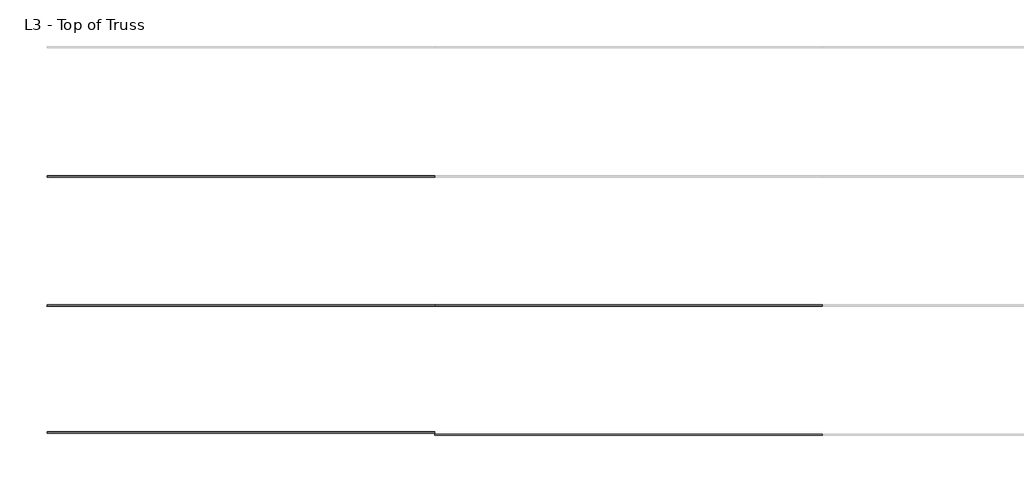
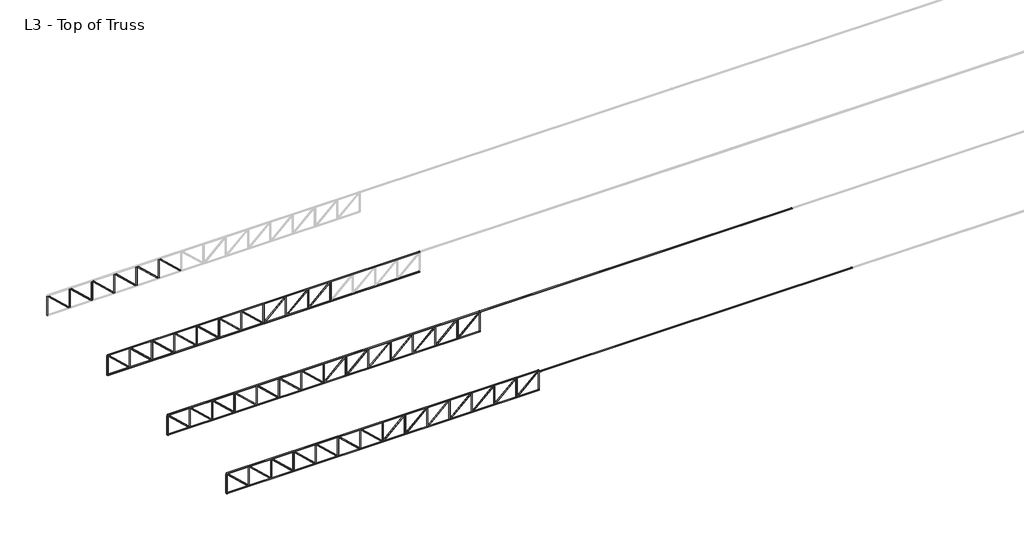
# One storey, part 1 of 2: 99 beams.
"""IFC4 building model written with IfcOpenShell, lengths in millimetres."""

import ifcopenshell
import ifcopenshell.guid

model = None  # the IFC model being written
_history = None  # IfcOwnerHistory: only IFC2X3 demands one
_inside = {}  # id of a spatial element -> (the spatial element, [elements in it])
_under = {}  # id of a project, library or spatial element -> (it, [spatial elements below it])
_declared = {}  # id of a project -> (the project, [libraries it declares])
_typed = {}  # id of a type object -> (the type object, [elements of that type])
_made_of = {}  # id of a material, layer set ... -> (it, [elements and type objects made of it])


def new_model(schema):
    """Start an empty IFC model of exactly this schema.

    Asked for "IFC4X3", IfcOpenShell would pick the latest addendum, in which some entities
    have other attributes; the version numbers below select the first issue.
    IFC2X3 requires an IfcOwnerHistory on every rooted entity: one is made here for all.
    """
    global model, _history
    if schema == "IFC4X3":
        model = ifcopenshell.file(schema_version=(4, 3, 0, 0))
    else:
        model = ifcopenshell.file(schema=schema)
    _inside.clear()
    _under.clear()
    _declared.clear()
    _typed.clear()
    _made_of.clear()
    _history = None
    if model.schema == "IFC2X3":
        org = make("IfcOrganization", Name="unknown")
        user = make(
            "IfcPersonAndOrganization",
            ThePerson=make("IfcPerson", FamilyName="unknown"),
            TheOrganization=org,
        )
        app = make(
            "IfcApplication",
            ApplicationDeveloper=org,
            Version="unknown",
            ApplicationFullName="unknown",
            ApplicationIdentifier="unknown",
        )
        _history = make(
            "IfcOwnerHistory",
            OwningUser=user,
            OwningApplication=app,
            ChangeAction="ADDED",
            CreationDate=0,
        )
    return model


def make(cls, **values):
    """One entity of the class cls with the attributes given. An attribute that is None is left unset."""
    return model.create_entity(
        cls, **{name: value for name, value in values.items() if value is not None}
    )


def rooted(cls, **values):
    """An entity with a GlobalId (a new one), such as an element, a storey or a relation."""
    return make(cls, GlobalId=ifcopenshell.guid.new(), OwnerHistory=_history, **values)


def si_unit(unit_type, name, prefix=None):
    """IfcSIUnit, for example si_unit("LENGTHUNIT", "METRE", prefix="MILLI")."""
    return make("IfcSIUnit", UnitType=unit_type, Prefix=prefix, Name=name)


def assignment(units):
    """IfcUnitAssignment: the units of a project."""
    return None if units is None else make("IfcUnitAssignment", Units=units)


def point(xyz):
    """IfcCartesianPoint."""
    return None if xyz is None else make("IfcCartesianPoint", Coordinates=xyz)


def direction(xyz):
    """IfcDirection."""
    return None if xyz is None else make("IfcDirection", DirectionRatios=xyz)


def frame(location, z_axis=None, x_axis=None):
    """IfcAxis2Placement3D, a coordinate frame: its origin and axes. An axis left out is left unset."""
    return make(
        "IfcAxis2Placement3D",
        Location=point(location),
        Axis=direction(z_axis),
        RefDirection=direction(x_axis),
    )


def frame_2d(location, x_axis=None):
    """IfcAxis2Placement2D, a coordinate frame in the plane: its origin and x axis."""
    return make(
        "IfcAxis2Placement2D", Location=point(location), RefDirection=direction(x_axis)
    )


def origin():
    """The frame at (0, 0, 0) with its axes left unset."""
    return frame((0.0, 0.0, 0.0))


def origin_2d():
    """The frame at (0, 0) in the plane with its x axis left unset."""
    return frame_2d((0.0, 0.0))


def place(relative_to, where):
    """IfcLocalPlacement: puts the frame where relative to a parent placement (None: the world)."""
    return make(
        "IfcLocalPlacement", PlacementRelTo=relative_to, RelativePlacement=where
    )


def context(
    kind, dimensions, precision=None, world=None, true_north=None, identifier=None
):
    """IfcGeometricRepresentationContext, for example the 3D "Model" context."""
    return make(
        "IfcGeometricRepresentationContext",
        ContextIdentifier=identifier,
        ContextType=kind,
        CoordinateSpaceDimension=dimensions,
        Precision=precision,
        WorldCoordinateSystem=world,
        TrueNorth=true_north,
    )


def project(units=None, contexts=None):
    """IfcProject with its units and contexts."""
    return rooted(
        "IfcProject",
        Name="project",
        RepresentationContexts=contexts,
        UnitsInContext=assignment(units),
    )


def spatial(cls, under=None, at=None, **own):
    """A site, building, storey or space (cls), placed at a placement, below another one or the project."""
    s = rooted(cls, ObjectPlacement=at, **own)
    if under is not None:
        _under.setdefault(under.id(), (under, []))[1].append(s)
    return s


def circle_curve(where, radius):
    """IfcCircle in the frame where."""
    return make("IfcCircle", Position=where, Radius=radius)


def trimmed(basis, trim1, trim2, sense, master):
    """IfcTrimmedCurve: the piece of a basis curve between two trims."""
    return make(
        "IfcTrimmedCurve",
        BasisCurve=basis,
        Trim1=trim1,
        Trim2=trim2,
        SenseAgreement=sense,
        MasterRepresentation=master,
    )


def segment(curve, same_sense, transition):
    """IfcCompositeCurveSegment."""
    return make(
        "IfcCompositeCurveSegment",
        Transition=transition,
        SameSense=same_sense,
        ParentCurve=curve,
    )


def composite_curve(segments, self_intersect=None):
    """IfcCompositeCurve: segments joined end to end."""
    return make("IfcCompositeCurve", Segments=segments, SelfIntersect=self_intersect)


def outline(outer, holes=None, kind="AREA"):
    """IfcArbitraryClosedProfileDef: a profile drawn as a closed curve; with holes, ...WithVoids."""
    if holes is None:
        return make("IfcArbitraryClosedProfileDef", ProfileType=kind, OuterCurve=outer)
    return make(
        "IfcArbitraryProfileDefWithVoids",
        ProfileType=kind,
        OuterCurve=outer,
        InnerCurves=holes,
    )


def extrude(swept, where, along, depth):
    """IfcExtrudedAreaSolid: the profile swept, set in the frame where, extruded along a direction by depth."""
    return make(
        "IfcExtrudedAreaSolid",
        SweptArea=swept,
        Position=where,
        ExtrudedDirection=direction(along),
        Depth=depth,
    )


def shape(context_of_items, identifier, shape_type, items):
    """IfcShapeRepresentation: the items that make up one representation, for example the "Body"."""
    return make(
        "IfcShapeRepresentation",
        ContextOfItems=context_of_items,
        RepresentationIdentifier=identifier,
        RepresentationType=shape_type,
        Items=items,
    )


def source(mapping_origin, context_of_items, identifier, shape_type, items):
    """IfcRepresentationMap: a shape defined once, which mapped items show again and again."""
    return make(
        "IfcRepresentationMap",
        MappingOrigin=mapping_origin,
        MappedRepresentation=shape(context_of_items, identifier, shape_type, items),
    )


def transform(
    local_origin,
    x_axis=None,
    y_axis=None,
    z_axis=None,
    scale=None,
    scale2=None,
    scale3=None,
    uniform=True,
):
    """IfcCartesianTransformationOperator3D, or its non-uniform kind. x_axis, y_axis, z_axis: its Axis1, 2, 3."""
    if uniform:
        return make(
            "IfcCartesianTransformationOperator3D",
            Axis1=direction(x_axis),
            Axis2=direction(y_axis),
            LocalOrigin=point(local_origin),
            Scale=scale,
            Axis3=direction(z_axis),
        )
    return make(
        "IfcCartesianTransformationOperator3DnonUniform",
        Axis1=direction(x_axis),
        Axis2=direction(y_axis),
        LocalOrigin=point(local_origin),
        Scale=scale,
        Axis3=direction(z_axis),
        Scale2=scale2,
        Scale3=scale3,
    )


def mapped(mapping_source, mapping_target):
    """IfcMappedItem: shows the shape of a source again, moved by a transform."""
    return make(
        "IfcMappedItem", MappingSource=mapping_source, MappingTarget=mapping_target
    )


def made_of(thing, what):
    """Note that an element or type object is made of a material, layer set ...; save() writes the relation."""
    if what is not None:
        _made_of.setdefault(what.id(), (what, []))[1].append(thing)
    return thing


def element(
    cls,
    number,
    at=None,
    inside=None,
    cuts=None,
    type_object=None,
    material=None,
    context=None,
    identifier="Body",
    shape_type=None,
    held_by="IfcProductDefinitionShape",
    body=None,
    shapes=None,
    **own,
):
    """One element of the class cls, such as IfcWall. Its Tag is "e" and its number.

    at: its placement. inside: the storey or other place that contains it. cuts: it is an
    opening in that element (IfcRelVoidsElement). A single representation is given by context,
    identifier, shape_type and body (its items); several are given by shapes. held_by: the class
    of the entity that holds the representations. save() writes the other relations.
    """
    e = rooted(cls, Tag="e%d" % number, ObjectPlacement=at, **own)
    if body is not None:
        shapes = [shape(context, identifier, shape_type, body)]
    if shapes is not None:
        e.Representation = make(held_by, Representations=shapes)
    if inside is not None:
        _inside.setdefault(inside.id(), (inside, []))[1].append(e)
    if cuts is not None:
        rooted(
            "IfcRelVoidsElement", RelatingBuildingElement=cuts, RelatedOpeningElement=e
        )
    if type_object is not None:
        _typed.setdefault(type_object.id(), (type_object, []))[1].append(e)
    return made_of(e, material)


def aggregate(whole, parts):
    """IfcRelAggregates: a whole, such as a stair, and the parts it consists of."""
    return rooted("IfcRelAggregates", RelatingObject=whole, RelatedObjects=parts)


def save(model, path):
    """Write the relations noted so far, then the file.

    IfcRelAggregates (storeys below a building ...), IfcRelContainedInSpatialStructure (elements
    in a storey), IfcRelDefinesByType, IfcRelAssociatesMaterial and IfcRelDeclares: one each for
    every whole, place, type object, material and project.
    """
    for whole, parts in _under.values():
        aggregate(whole, parts)
    for where, things in _inside.values():
        rooted(
            "IfcRelContainedInSpatialStructure",
            RelatedElements=things,
            RelatingStructure=where,
        )
    for kind, things in _typed.values():
        rooted("IfcRelDefinesByType", RelatedObjects=things, RelatingType=kind)
    for what, things in _made_of.values():
        rooted("IfcRelAssociatesMaterial", RelatedObjects=things, RelatingMaterial=what)
    for by, libraries in _declared.values():
        rooted("IfcRelDeclares", RelatingContext=by, RelatedDefinitions=libraries)
    model.write(path)


def circular_hollow_sections_chs60_3x5_c94bd862(model_context):
    return source(origin(), model_context, "Body", "SweptSolid", [
        extrude(outline(composite_curve([segment(trimmed(circle_curve(origin_2d(), 30.15), [point((-30.15, 0.0))], [point((30.15, 0.0))], False, "CARTESIAN"), True, "CONTINUOUS"), segment(trimmed(circle_curve(origin_2d(), 30.15), [point((30.15, 0.0))], [point((-30.15, 0.0))], False, "CARTESIAN"), True, "CONTINUOUS")], self_intersect=False), holes=[composite_curve([segment(trimmed(circle_curve(origin_2d(), 25.15), [point((25.15, 0.0))], [point((-25.15, 0.0))], True, "CARTESIAN"), True, "CONTINUOUS"), segment(trimmed(circle_curve(origin_2d(), 25.15), [point((-25.15, 0.0))], [point((25.15, 0.0))], True, "CARTESIAN"), True, "CONTINUOUS")], self_intersect=False)]), frame((-557.0, 0.0, 0.0), z_axis=(1.0, 0.0, 0.0), x_axis=(0.0, 1.0, 0.0)), (0.0, 0.0, 1.0), 1114.0),
    ])


def circular_hollow_sections_chs60_3x5_b8a643cb(model_context):
    return source(origin(), model_context, "Body", "SweptSolid", [
        extrude(outline(composite_curve([segment(trimmed(circle_curve(origin_2d(), 30.15), [point((-30.15, 0.0))], [point((30.15, 0.0))], False, "CARTESIAN"), True, "CONTINUOUS"), segment(trimmed(circle_curve(origin_2d(), 30.15), [point((30.15, 0.0))], [point((-30.15, 0.0))], False, "CARTESIAN"), True, "CONTINUOUS")], self_intersect=False), holes=[composite_curve([segment(trimmed(circle_curve(origin_2d(), 25.15), [point((25.15, 0.0))], [point((-25.15, 0.0))], True, "CARTESIAN"), True, "CONTINUOUS"), segment(trimmed(circle_curve(origin_2d(), 25.15), [point((-25.15, 0.0))], [point((25.15, 0.0))], True, "CARTESIAN"), True, "CONTINUOUS")], self_intersect=False)]), frame((-790.0, 0.0, 0.0), z_axis=(1.0, 0.0, 0.0), x_axis=(0.0, 1.0, 0.0)), (0.0, 0.0, 1.0), 1580.0),
    ])


def circular_hollow_sections_chs60_3x5_ee2473de(model_context):
    return source(origin(), model_context, "Body", "SweptSolid", [
        extrude(outline(composite_curve([segment(trimmed(circle_curve(origin_2d(), 30.15), [point((-30.15, 0.0))], [point((30.15, 0.0))], False, "CARTESIAN"), True, "CONTINUOUS"), segment(trimmed(circle_curve(origin_2d(), 30.15), [point((30.15, 0.0))], [point((-30.15, 0.0))], False, "CARTESIAN"), True, "CONTINUOUS")], self_intersect=False), holes=[composite_curve([segment(trimmed(circle_curve(origin_2d(), 25.15), [point((25.15, 0.0))], [point((-25.15, 0.0))], True, "CARTESIAN"), True, "CONTINUOUS"), segment(trimmed(circle_curve(origin_2d(), 25.15), [point((-25.15, 0.0))], [point((25.15, 0.0))], True, "CARTESIAN"), True, "CONTINUOUS")], self_intersect=False)]), frame((-9000.0, 0.0, 0.0), z_axis=(1.0, 0.0, 0.0), x_axis=(0.0, 1.0, 0.0)), (0.0, 0.0, 1.0), 18000.0),
    ])


def circular_hollow_sections_chs60_3x5_7809bf4e(model_context):
    return source(origin(), model_context, "Body", "SweptSolid", [
        extrude(outline(composite_curve([segment(trimmed(circle_curve(origin_2d(), 30.15), [point((-30.15, 0.0))], [point((30.15, 0.0))], False, "CARTESIAN"), True, "CONTINUOUS"), segment(trimmed(circle_curve(origin_2d(), 30.15), [point((30.15, 0.0))], [point((-30.15, 0.0))], False, "CARTESIAN"), True, "CONTINUOUS")], self_intersect=False), holes=[composite_curve([segment(trimmed(circle_curve(origin_2d(), 25.15), [point((25.15, 0.0))], [point((-25.15, 0.0))], True, "CARTESIAN"), True, "CONTINUOUS"), segment(trimmed(circle_curve(origin_2d(), 25.15), [point((-25.15, 0.0))], [point((25.15, 0.0))], True, "CARTESIAN"), True, "CONTINUOUS")], self_intersect=False)]), frame((-600.0, 0.0, 0.0), z_axis=(1.0, 0.0, 0.0), x_axis=(0.0, 1.0, 0.0)), (0.0, 0.0, 1.0), 1157.0),
    ])


model = new_model("IFC4")

# Units and contexts
model_context = context("Model", 3, world=origin())
ifc_project = project(units=[si_unit("LENGTHUNIT", "METRE", prefix="MILLI")], contexts=[model_context])

# Site, building, storey
site = spatial("IfcSite", under=ifc_project)
building = spatial("IfcBuilding", under=site)
storey = spatial("IfcBuildingStorey", under=building, Name="L3 - Top of Truss", Elevation=7800.0)

# Beams
placement = place(None, origin())
circular_hollow_sections_chs60_3x5_shape = circular_hollow_sections_chs60_3x5_c94bd862(model_context)
element("IfcBeam", 1, ObjectType="Circular Hollow Sections : CHS60.3x5", at=placement, inside=storey, context=model_context, shape_type="MappedRepresentation", body=[
    mapped(circular_hollow_sections_chs60_3x5_shape, transform((-5853.84106, -5058.7619082, 7200.0), x_axis=(0.0, 0.0, 1.0), y_axis=(0.0, -1.0, 0.0), z_axis=(1.0, 0.0, 0.0))),
])
element("IfcBeam", 2, ObjectType="Circular Hollow Sections : CHS60.3x5", at=placement, inside=storey, context=model_context, shape_type="MappedRepresentation", body=[
    mapped(circular_hollow_sections_chs60_3x5_shape, transform((-4568.1267743, -5058.7619082, 7200.0), x_axis=(0.0, 0.0, 1.0), y_axis=(0.0, -1.0, 0.0), z_axis=(1.0, 0.0, 0.0))),
])
element("IfcBeam", 3, ObjectType="Circular Hollow Sections : CHS60.3x5", at=placement, inside=storey, context=model_context, shape_type="MappedRepresentation", body=[
    mapped(circular_hollow_sections_chs60_3x5_shape, transform((-3282.4124885, -5058.7619082, 7200.0), x_axis=(0.0, 0.0, 1.0), y_axis=(0.0, -1.0, 0.0), z_axis=(1.0, 0.0, 0.0))),
])
element("IfcBeam", 4, ObjectType="Circular Hollow Sections : CHS60.3x5", at=placement, inside=storey, context=model_context, shape_type="MappedRepresentation", body=[
    mapped(circular_hollow_sections_chs60_3x5_shape, transform((-1996.6982028, -5058.7619082, 7200.0), x_axis=(0.0, 0.0, 1.0), y_axis=(0.0, -1.0, 0.0), z_axis=(1.0, 0.0, 0.0))),
])
element("IfcBeam", 5, ObjectType="Circular Hollow Sections : CHS60.3x5", at=placement, inside=storey, context=model_context, shape_type="MappedRepresentation", body=[
    mapped(circular_hollow_sections_chs60_3x5_shape, transform((-710.9839171, -5058.7619082, 7200.0), x_axis=(0.0, 0.0, 1.0), y_axis=(0.0, -1.0, 0.0), z_axis=(1.0, 0.0, 0.0))),
])
element("IfcBeam", 6, ObjectType="Circular Hollow Sections : CHS60.3x5", at=placement, inside=storey, context=model_context, shape_type="MappedRepresentation", body=[
    mapped(circular_hollow_sections_chs60_3x5_shape, transform((-5853.84106, -11058.7619082, 7200.0), x_axis=(0.0, 0.0, 1.0), y_axis=(0.0, -1.0, 0.0), z_axis=(1.0, 0.0, 0.0))),
])
element("IfcBeam", 7, ObjectType="Circular Hollow Sections : CHS60.3x5", at=placement, inside=storey, context=model_context, shape_type="MappedRepresentation", body=[
    mapped(circular_hollow_sections_chs60_3x5_shape, transform((-4568.1267743, -11058.7619082, 7200.0), x_axis=(0.0, 0.0, 1.0), y_axis=(0.0, -1.0, 0.0), z_axis=(1.0, 0.0, 0.0))),
])
element("IfcBeam", 8, ObjectType="Circular Hollow Sections : CHS60.3x5", at=placement, inside=storey, context=model_context, shape_type="MappedRepresentation", body=[
    mapped(circular_hollow_sections_chs60_3x5_shape, transform((-3282.4124885, -11058.7619082, 7200.0), x_axis=(0.0, 0.0, 1.0), y_axis=(0.0, -1.0, 0.0), z_axis=(1.0, 0.0, 0.0))),
])
element("IfcBeam", 9, ObjectType="Circular Hollow Sections : CHS60.3x5", at=placement, inside=storey, context=model_context, shape_type="MappedRepresentation", body=[
    mapped(circular_hollow_sections_chs60_3x5_shape, transform((5717.5875115, -11058.7619082, 7200.0), x_axis=(0.0, 0.0, 1.0), y_axis=(0.0, -1.0, 0.0), z_axis=(1.0, 0.0, 0.0))),
])
element("IfcBeam", 10, ObjectType="Circular Hollow Sections : CHS60.3x5", at=placement, inside=storey, context=model_context, shape_type="MappedRepresentation", body=[
    mapped(circular_hollow_sections_chs60_3x5_shape, transform((4431.8732257, -11058.7619082, 7200.0), x_axis=(0.0, 0.0, 1.0), y_axis=(0.0, -1.0, 0.0), z_axis=(1.0, 0.0, 0.0))),
])
element("IfcBeam", 11, ObjectType="Circular Hollow Sections : CHS60.3x5", at=placement, inside=storey, context=model_context, shape_type="MappedRepresentation", body=[
    mapped(circular_hollow_sections_chs60_3x5_shape, transform((3146.15894, -11058.7619082, 7200.0), x_axis=(0.0, 0.0, 1.0), y_axis=(0.0, -1.0, 0.0), z_axis=(1.0, 0.0, 0.0))),
])
element("IfcBeam", 12, ObjectType="Circular Hollow Sections : CHS60.3x5", at=placement, inside=storey, context=model_context, shape_type="MappedRepresentation", body=[
    mapped(circular_hollow_sections_chs60_3x5_shape, transform((-1996.6982028, -11058.7619082, 7200.0), x_axis=(0.0, 0.0, 1.0), y_axis=(0.0, -1.0, 0.0), z_axis=(1.0, 0.0, 0.0))),
])
element("IfcBeam", 13, ObjectType="Circular Hollow Sections : CHS60.3x5", at=placement, inside=storey, context=model_context, shape_type="MappedRepresentation", body=[
    mapped(circular_hollow_sections_chs60_3x5_shape, transform((-710.9839171, -11058.7619082, 7200.0), x_axis=(0.0, 0.0, 1.0), y_axis=(0.0, -1.0, 0.0), z_axis=(1.0, 0.0, 0.0))),
])
element("IfcBeam", 14, ObjectType="Circular Hollow Sections : CHS60.3x5", at=placement, inside=storey, context=model_context, shape_type="MappedRepresentation", body=[
    mapped(circular_hollow_sections_chs60_3x5_shape, transform((574.7303686, -11058.7619082, 7200.0), x_axis=(0.0, 0.0, 1.0), y_axis=(0.0, -1.0, 0.0), z_axis=(1.0, 0.0, 0.0))),
])
element("IfcBeam", 15, ObjectType="Circular Hollow Sections : CHS60.3x5", at=placement, inside=storey, context=model_context, shape_type="MappedRepresentation", body=[
    mapped(circular_hollow_sections_chs60_3x5_shape, transform((1860.4446543, -11058.7619082, 7200.0), x_axis=(0.0, 0.0, 1.0), y_axis=(0.0, -1.0, 0.0), z_axis=(1.0, 0.0, 0.0))),
])
element("IfcBeam", 16, ObjectType="Circular Hollow Sections : CHS60.3x5", at=placement, inside=storey, context=model_context, shape_type="MappedRepresentation", body=[
    mapped(circular_hollow_sections_chs60_3x5_shape, transform((9574.7303686, -17058.7619082, 7200.0), x_axis=(0.0, 0.0, 1.0), y_axis=(0.0, -1.0, 0.0), z_axis=(1.0, 0.0, 0.0))),
])
element("IfcBeam", 17, ObjectType="Circular Hollow Sections : CHS60.3x5", at=placement, inside=storey, context=model_context, shape_type="MappedRepresentation", body=[
    mapped(circular_hollow_sections_chs60_3x5_shape, transform((-5853.84106, -17058.7619082, 7200.0), x_axis=(0.0, 0.0, 1.0), y_axis=(0.0, -1.0, 0.0), z_axis=(1.0, 0.0, 0.0))),
])
element("IfcBeam", 18, ObjectType="Circular Hollow Sections : CHS60.3x5", at=placement, inside=storey, context=model_context, shape_type="MappedRepresentation", body=[
    mapped(circular_hollow_sections_chs60_3x5_shape, transform((8289.0160829, -17058.7619082, 7200.0), x_axis=(0.0, 0.0, 1.0), y_axis=(0.0, -1.0, 0.0), z_axis=(1.0, 0.0, 0.0))),
])
element("IfcBeam", 19, ObjectType="Circular Hollow Sections : CHS60.3x5", at=placement, inside=storey, context=model_context, shape_type="MappedRepresentation", body=[
    mapped(circular_hollow_sections_chs60_3x5_shape, transform((-4568.1267743, -17058.7619082, 7200.0), x_axis=(0.0, 0.0, 1.0), y_axis=(0.0, -1.0, 0.0), z_axis=(1.0, 0.0, 0.0))),
])
element("IfcBeam", 20, ObjectType="Circular Hollow Sections : CHS60.3x5", at=placement, inside=storey, context=model_context, shape_type="MappedRepresentation", body=[
    mapped(circular_hollow_sections_chs60_3x5_shape, transform((7003.3017972, -17058.7619082, 7200.0), x_axis=(0.0, 0.0, 1.0), y_axis=(0.0, -1.0, 0.0), z_axis=(1.0, 0.0, 0.0))),
])
element("IfcBeam", 21, ObjectType="Circular Hollow Sections : CHS60.3x5", at=placement, inside=storey, context=model_context, shape_type="MappedRepresentation", body=[
    mapped(circular_hollow_sections_chs60_3x5_shape, transform((-3282.4124885, -17058.7619082, 7200.0), x_axis=(0.0, 0.0, 1.0), y_axis=(0.0, -1.0, 0.0), z_axis=(1.0, 0.0, 0.0))),
])
element("IfcBeam", 22, ObjectType="Circular Hollow Sections : CHS60.3x5", at=placement, inside=storey, context=model_context, shape_type="MappedRepresentation", body=[
    mapped(circular_hollow_sections_chs60_3x5_shape, transform((5717.5875115, -17058.7619082, 7200.0), x_axis=(0.0, 0.0, 1.0), y_axis=(0.0, -1.0, 0.0), z_axis=(1.0, 0.0, 0.0))),
])
element("IfcBeam", 23, ObjectType="Circular Hollow Sections : CHS60.3x5", at=placement, inside=storey, context=model_context, shape_type="MappedRepresentation", body=[
    mapped(circular_hollow_sections_chs60_3x5_shape, transform((4431.8732257, -17058.7619082, 7200.0), x_axis=(0.0, 0.0, 1.0), y_axis=(0.0, -1.0, 0.0), z_axis=(1.0, 0.0, 0.0))),
])
element("IfcBeam", 24, ObjectType="Circular Hollow Sections : CHS60.3x5", at=placement, inside=storey, context=model_context, shape_type="MappedRepresentation", body=[
    mapped(circular_hollow_sections_chs60_3x5_shape, transform((3146.15894, -17058.7619082, 7200.0), x_axis=(0.0, 0.0, 1.0), y_axis=(0.0, -1.0, 0.0), z_axis=(1.0, 0.0, 0.0))),
])
element("IfcBeam", 25, ObjectType="Circular Hollow Sections : CHS60.3x5", at=placement, inside=storey, context=model_context, shape_type="MappedRepresentation", body=[
    mapped(circular_hollow_sections_chs60_3x5_shape, transform((-1996.6982028, -17058.7619082, 7200.0), x_axis=(0.0, 0.0, 1.0), y_axis=(0.0, -1.0, 0.0), z_axis=(1.0, 0.0, 0.0))),
])
element("IfcBeam", 26, ObjectType="Circular Hollow Sections : CHS60.3x5", at=placement, inside=storey, context=model_context, shape_type="MappedRepresentation", body=[
    mapped(circular_hollow_sections_chs60_3x5_shape, transform((-710.9839171, -17058.7619082, 7200.0), x_axis=(0.0, 0.0, 1.0), y_axis=(0.0, -1.0, 0.0), z_axis=(1.0, 0.0, 0.0))),
])
element("IfcBeam", 27, ObjectType="Circular Hollow Sections : CHS60.3x5", at=placement, inside=storey, context=model_context, shape_type="MappedRepresentation", body=[
    mapped(circular_hollow_sections_chs60_3x5_shape, transform((574.7303686, -17058.7619082, 7200.0), x_axis=(0.0, 0.0, 1.0), y_axis=(0.0, -1.0, 0.0), z_axis=(1.0, 0.0, 0.0))),
])
element("IfcBeam", 28, ObjectType="Circular Hollow Sections : CHS60.3x5", at=placement, inside=storey, context=model_context, shape_type="MappedRepresentation", body=[
    mapped(circular_hollow_sections_chs60_3x5_shape, transform((1860.4446543, -17058.7619082, 7200.0), x_axis=(0.0, 0.0, 1.0), y_axis=(0.0, -1.0, 0.0), z_axis=(1.0, 0.0, 0.0))),
])
element("IfcBeam", 29, ObjectType="Circular Hollow Sections : CHS60.3x5", at=placement, inside=storey, context=model_context, shape_type="MappedRepresentation", body=[
    mapped(circular_hollow_sections_chs60_3x5_shape, transform((9574.7303686, -22948.7619082, 7200.0), x_axis=(0.0, 0.0, 1.0), y_axis=(0.0, -1.0, 0.0), z_axis=(1.0, 0.0, 0.0))),
])
element("IfcBeam", 30, ObjectType="Circular Hollow Sections : CHS60.3x5", at=placement, inside=storey, context=model_context, shape_type="MappedRepresentation", body=[
    mapped(circular_hollow_sections_chs60_3x5_shape, transform((-5853.84106, -22948.7619082, 7200.0), x_axis=(0.0, 0.0, 1.0), y_axis=(0.0, -1.0, 0.0), z_axis=(1.0, 0.0, 0.0))),
])
element("IfcBeam", 31, ObjectType="Circular Hollow Sections : CHS60.3x5", at=placement, inside=storey, context=model_context, shape_type="MappedRepresentation", body=[
    mapped(circular_hollow_sections_chs60_3x5_shape, transform((8289.0160829, -22948.7619082, 7200.0), x_axis=(0.0, 0.0, 1.0), y_axis=(0.0, -1.0, 0.0), z_axis=(1.0, 0.0, 0.0))),
])
element("IfcBeam", 32, ObjectType="Circular Hollow Sections : CHS60.3x5", at=placement, inside=storey, context=model_context, shape_type="MappedRepresentation", body=[
    mapped(circular_hollow_sections_chs60_3x5_shape, transform((-4568.1267743, -22948.7619082, 7200.0), x_axis=(0.0, 0.0, 1.0), y_axis=(0.0, -1.0, 0.0), z_axis=(1.0, 0.0, 0.0))),
])
element("IfcBeam", 33, ObjectType="Circular Hollow Sections : CHS60.3x5", at=placement, inside=storey, context=model_context, shape_type="MappedRepresentation", body=[
    mapped(circular_hollow_sections_chs60_3x5_shape, transform((7003.3017972, -22948.7619082, 7200.0), x_axis=(0.0, 0.0, 1.0), y_axis=(0.0, -1.0, 0.0), z_axis=(1.0, 0.0, 0.0))),
])
element("IfcBeam", 34, ObjectType="Circular Hollow Sections : CHS60.3x5", at=placement, inside=storey, context=model_context, shape_type="MappedRepresentation", body=[
    mapped(circular_hollow_sections_chs60_3x5_shape, transform((-3282.4124885, -22948.7619082, 7200.0), x_axis=(0.0, 0.0, 1.0), y_axis=(0.0, -1.0, 0.0), z_axis=(1.0, 0.0, 0.0))),
])
element("IfcBeam", 35, ObjectType="Circular Hollow Sections : CHS60.3x5", at=placement, inside=storey, context=model_context, shape_type="MappedRepresentation", body=[
    mapped(circular_hollow_sections_chs60_3x5_shape, transform((5717.5875115, -22948.7619082, 7200.0), x_axis=(0.0, 0.0, 1.0), y_axis=(0.0, -1.0, 0.0), z_axis=(1.0, 0.0, 0.0))),
])
element("IfcBeam", 36, ObjectType="Circular Hollow Sections : CHS60.3x5", at=placement, inside=storey, context=model_context, shape_type="MappedRepresentation", body=[
    mapped(circular_hollow_sections_chs60_3x5_shape, transform((4431.8732257, -22948.7619082, 7200.0), x_axis=(0.0, 0.0, 1.0), y_axis=(0.0, -1.0, 0.0), z_axis=(1.0, 0.0, 0.0))),
])
element("IfcBeam", 37, ObjectType="Circular Hollow Sections : CHS60.3x5", at=placement, inside=storey, context=model_context, shape_type="MappedRepresentation", body=[
    mapped(circular_hollow_sections_chs60_3x5_shape, transform((10860.4446543, -22948.7619082, 7200.0), x_axis=(0.0, 0.0, 1.0), y_axis=(0.0, -1.0, 0.0), z_axis=(1.0, 0.0, 0.0))),
])
element("IfcBeam", 38, ObjectType="Circular Hollow Sections : CHS60.3x5", at=placement, inside=storey, context=model_context, shape_type="MappedRepresentation", body=[
    mapped(circular_hollow_sections_chs60_3x5_shape, transform((3146.15894, -22948.7619082, 7200.0), x_axis=(0.0, 0.0, 1.0), y_axis=(0.0, -1.0, 0.0), z_axis=(1.0, 0.0, 0.0))),
])
element("IfcBeam", 39, ObjectType="Circular Hollow Sections : CHS60.3x5", at=placement, inside=storey, context=model_context, shape_type="MappedRepresentation", body=[
    mapped(circular_hollow_sections_chs60_3x5_shape, transform((-1996.6982028, -22948.7619082, 7200.0), x_axis=(0.0, 0.0, 1.0), y_axis=(0.0, -1.0, 0.0), z_axis=(1.0, 0.0, 0.0))),
])
element("IfcBeam", 40, ObjectType="Circular Hollow Sections : CHS60.3x5", at=placement, inside=storey, context=model_context, shape_type="MappedRepresentation", body=[
    mapped(circular_hollow_sections_chs60_3x5_shape, transform((-710.9839171, -22948.7619082, 7200.0), x_axis=(0.0, 0.0, 1.0), y_axis=(0.0, -1.0, 0.0), z_axis=(1.0, 0.0, 0.0))),
])
element("IfcBeam", 41, ObjectType="Circular Hollow Sections : CHS60.3x5", at=placement, inside=storey, context=model_context, shape_type="MappedRepresentation", body=[
    mapped(circular_hollow_sections_chs60_3x5_shape, transform((-7139.5553457, -22948.7619082, 7200.0), x_axis=(0.0, 0.0, 1.0), y_axis=(0.0, -1.0, 0.0), z_axis=(1.0, 0.0, 0.0))),
])
element("IfcBeam", 42, ObjectType="Circular Hollow Sections : CHS60.3x5", at=placement, inside=storey, context=model_context, shape_type="MappedRepresentation", body=[
    mapped(circular_hollow_sections_chs60_3x5_shape, transform((574.7303686, -22948.7619082, 7200.0), x_axis=(0.0, 0.0, 1.0), y_axis=(0.0, -1.0, 0.0), z_axis=(1.0, 0.0, 0.0))),
])
element("IfcBeam", 43, ObjectType="Circular Hollow Sections : CHS60.3x5", at=placement, inside=storey, context=model_context, shape_type="MappedRepresentation", body=[
    mapped(circular_hollow_sections_chs60_3x5_shape, transform((1860.4446543, -22948.7619082, 7200.0), x_axis=(0.0, 0.0, 1.0), y_axis=(0.0, -1.0, 0.0), z_axis=(1.0, 0.0, 0.0))),
])
circular_hollow_sections_chs60_3x5_2_shape = circular_hollow_sections_chs60_3x5_b8a643cb(model_context)
element("IfcBeam", 44, ObjectType="Circular Hollow Sections : CHS60.3x5", at=placement, inside=storey, context=model_context, shape_type="MappedRepresentation", body=[
    mapped(circular_hollow_sections_chs60_3x5_2_shape, transform((-5210.9839171, -5058.7619082, 7200.0), x_axis=(0.7310552682428689, 0.0, -0.6823182503600113), y_axis=(0.0, -1.0, 0.0), z_axis=(-0.6823182503600113, 0.0, -0.7310552682428689))),
])
element("IfcBeam", 45, ObjectType="Circular Hollow Sections : CHS60.3x5", at=placement, inside=storey, context=model_context, shape_type="MappedRepresentation", body=[
    mapped(circular_hollow_sections_chs60_3x5_2_shape, transform((-3925.2696314, -5058.7619082, 7200.0), x_axis=(0.7310552682428689, 0.0, -0.6823182503600113), y_axis=(0.0, -1.0, 0.0), z_axis=(-0.6823182503600113, 0.0, -0.7310552682428689))),
])
element("IfcBeam", 46, ObjectType="Circular Hollow Sections : CHS60.3x5", at=placement, inside=storey, context=model_context, shape_type="MappedRepresentation", body=[
    mapped(circular_hollow_sections_chs60_3x5_2_shape, transform((-2639.5553457, -5058.7619082, 7200.0), x_axis=(0.7310552682428689, 0.0, -0.6823182503600113), y_axis=(0.0, -1.0, 0.0), z_axis=(-0.6823182503600113, 0.0, -0.7310552682428689))),
])
element("IfcBeam", 47, ObjectType="Circular Hollow Sections : CHS60.3x5", at=placement, inside=storey, context=model_context, shape_type="MappedRepresentation", body=[
    mapped(circular_hollow_sections_chs60_3x5_2_shape, transform((-1353.84106, -5058.7619082, 7200.0), x_axis=(0.7310552682428689, 0.0, -0.6823182503600113), y_axis=(0.0, -1.0, 0.0), z_axis=(-0.6823182503600113, 0.0, -0.7310552682428689))),
])
element("IfcBeam", 48, ObjectType="Circular Hollow Sections : CHS60.3x5", at=placement, inside=storey, context=model_context, shape_type="MappedRepresentation", body=[
    mapped(circular_hollow_sections_chs60_3x5_2_shape, transform((-68.1267743, -5058.7619082, 7200.0), x_axis=(0.7310552682428689, 0.0, -0.6823182503600113), y_axis=(0.0, -1.0, 0.0), z_axis=(-0.6823182503600113, 0.0, -0.7310552682428689))),
])
element("IfcBeam", 49, ObjectType="Circular Hollow Sections : CHS60.3x5", at=placement, inside=storey, context=model_context, shape_type="MappedRepresentation", body=[
    mapped(circular_hollow_sections_chs60_3x5_2_shape, transform((-6496.6982028, -5058.7619082, 7200.0), x_axis=(0.7310552682428691, 0.0, -0.6823182503600111), y_axis=(0.0, -1.0, 0.0), z_axis=(-0.6823182503600111, 0.0, -0.7310552682428691))),
])
element("IfcBeam", 50, ObjectType="Circular Hollow Sections : CHS60.3x5", at=placement, inside=storey, context=model_context, shape_type="MappedRepresentation", body=[
    mapped(circular_hollow_sections_chs60_3x5_2_shape, transform((-5210.9839171, -11058.7619082, 7200.0), x_axis=(0.7310552682428689, 0.0, -0.6823182503600113), y_axis=(0.0, -1.0, 0.0), z_axis=(-0.6823182503600113, 0.0, -0.7310552682428689))),
])
element("IfcBeam", 51, ObjectType="Circular Hollow Sections : CHS60.3x5", at=placement, inside=storey, context=model_context, shape_type="MappedRepresentation", body=[
    mapped(circular_hollow_sections_chs60_3x5_2_shape, transform((-3925.2696314, -11058.7619082, 7200.0), x_axis=(0.7310552682428689, 0.0, -0.6823182503600113), y_axis=(0.0, -1.0, 0.0), z_axis=(-0.6823182503600113, 0.0, -0.7310552682428689))),
])
element("IfcBeam", 52, ObjectType="Circular Hollow Sections : CHS60.3x5", at=placement, inside=storey, context=model_context, shape_type="MappedRepresentation", body=[
    mapped(circular_hollow_sections_chs60_3x5_2_shape, transform((-2639.5553457, -11058.7619082, 7200.0), x_axis=(0.7310552682428689, 0.0, -0.6823182503600113), y_axis=(0.0, -1.0, 0.0), z_axis=(-0.6823182503600113, 0.0, -0.7310552682428689))),
])
element("IfcBeam", 53, ObjectType="Circular Hollow Sections : CHS60.3x5", at=placement, inside=storey, context=model_context, shape_type="MappedRepresentation", body=[
    mapped(circular_hollow_sections_chs60_3x5_2_shape, transform((5074.7303686, -11058.7619082, 7200.0), x_axis=(0.7310552682428691, 0.0, 0.6823182503600111), y_axis=(0.0, -1.0, 0.0), z_axis=(0.6823182503600111, 0.0, -0.7310552682428691))),
])
element("IfcBeam", 54, ObjectType="Circular Hollow Sections : CHS60.3x5", at=placement, inside=storey, context=model_context, shape_type="MappedRepresentation", body=[
    mapped(circular_hollow_sections_chs60_3x5_2_shape, transform((3789.0160829, -11058.7619082, 7200.0), x_axis=(0.7310552682428691, 0.0, 0.6823182503600111), y_axis=(0.0, -1.0, 0.0), z_axis=(0.6823182503600111, 0.0, -0.7310552682428691))),
])
element("IfcBeam", 55, ObjectType="Circular Hollow Sections : CHS60.3x5", at=placement, inside=storey, context=model_context, shape_type="MappedRepresentation", body=[
    mapped(circular_hollow_sections_chs60_3x5_2_shape, transform((2503.3017972, -11058.7619082, 7200.0), x_axis=(0.7310552682428691, 0.0, 0.682318250360011), y_axis=(0.0, -1.0, 0.0), z_axis=(0.682318250360011, 0.0, -0.7310552682428691))),
])
element("IfcBeam", 56, ObjectType="Circular Hollow Sections : CHS60.3x5", at=placement, inside=storey, context=model_context, shape_type="MappedRepresentation", body=[
    mapped(circular_hollow_sections_chs60_3x5_2_shape, transform((-1353.84106, -11058.7619082, 7200.0), x_axis=(0.7310552682428689, 0.0, -0.6823182503600113), y_axis=(0.0, -1.0, 0.0), z_axis=(-0.6823182503600113, 0.0, -0.7310552682428689))),
])
element("IfcBeam", 57, ObjectType="Circular Hollow Sections : CHS60.3x5", at=placement, inside=storey, context=model_context, shape_type="MappedRepresentation", body=[
    mapped(circular_hollow_sections_chs60_3x5_2_shape, transform((-68.1267743, -11058.7619082, 7200.0), x_axis=(0.7310552682428689, 0.0, -0.6823182503600113), y_axis=(0.0, -1.0, 0.0), z_axis=(-0.6823182503600113, 0.0, -0.7310552682428689))),
])
element("IfcBeam", 58, ObjectType="Circular Hollow Sections : CHS60.3x5", at=placement, inside=storey, context=model_context, shape_type="MappedRepresentation", body=[
    mapped(circular_hollow_sections_chs60_3x5_2_shape, transform((-6496.6982028, -11058.7619082, 7200.0), x_axis=(0.7310552682428688, 0.0, -0.6823182503600115), y_axis=(0.0, -1.0, 0.0), z_axis=(-0.6823182503600115, 0.0, -0.7310552682428688))),
])
element("IfcBeam", 59, ObjectType="Circular Hollow Sections : CHS60.3x5", at=placement, inside=storey, context=model_context, shape_type="MappedRepresentation", body=[
    mapped(circular_hollow_sections_chs60_3x5_2_shape, transform((1217.5875115, -11058.7619082, 7200.0), x_axis=(0.7310552682428689, 0.0, -0.6823182503600113), y_axis=(0.0, -1.0, 0.0), z_axis=(-0.6823182503600113, 0.0, -0.7310552682428689))),
])
element("IfcBeam", 60, ObjectType="Circular Hollow Sections : CHS60.3x5", at=placement, inside=storey, context=model_context, shape_type="MappedRepresentation", body=[
    mapped(circular_hollow_sections_chs60_3x5_2_shape, transform((8931.8732257, -17058.7619082, 7200.0), x_axis=(0.7310552682428691, 0.0, 0.6823182503600111), y_axis=(0.0, -1.0, 0.0), z_axis=(0.6823182503600111, 0.0, -0.7310552682428691))),
])
element("IfcBeam", 61, ObjectType="Circular Hollow Sections : CHS60.3x5", at=placement, inside=storey, context=model_context, shape_type="MappedRepresentation", body=[
    mapped(circular_hollow_sections_chs60_3x5_2_shape, transform((-5210.9839171, -17058.7619082, 7200.0), x_axis=(0.7310552682428689, 0.0, -0.6823182503600113), y_axis=(0.0, -1.0, 0.0), z_axis=(-0.6823182503600113, 0.0, -0.7310552682428689))),
])
element("IfcBeam", 62, ObjectType="Circular Hollow Sections : CHS60.3x5", at=placement, inside=storey, context=model_context, shape_type="MappedRepresentation", body=[
    mapped(circular_hollow_sections_chs60_3x5_2_shape, transform((7646.15894, -17058.7619082, 7200.0), x_axis=(0.7310552682428691, 0.0, 0.6823182503600111), y_axis=(0.0, -1.0, 0.0), z_axis=(0.6823182503600111, 0.0, -0.7310552682428691))),
])
element("IfcBeam", 63, ObjectType="Circular Hollow Sections : CHS60.3x5", at=placement, inside=storey, context=model_context, shape_type="MappedRepresentation", body=[
    mapped(circular_hollow_sections_chs60_3x5_2_shape, transform((-3925.2696314, -17058.7619082, 7200.0), x_axis=(0.7310552682428689, 0.0, -0.6823182503600113), y_axis=(0.0, -1.0, 0.0), z_axis=(-0.6823182503600113, 0.0, -0.7310552682428689))),
])
element("IfcBeam", 64, ObjectType="Circular Hollow Sections : CHS60.3x5", at=placement, inside=storey, context=model_context, shape_type="MappedRepresentation", body=[
    mapped(circular_hollow_sections_chs60_3x5_2_shape, transform((6360.4446543, -17058.7619082, 7200.0), x_axis=(0.7310552682428691, 0.0, 0.6823182503600111), y_axis=(0.0, -1.0, 0.0), z_axis=(0.6823182503600111, 0.0, -0.7310552682428691))),
])
element("IfcBeam", 65, ObjectType="Circular Hollow Sections : CHS60.3x5", at=placement, inside=storey, context=model_context, shape_type="MappedRepresentation", body=[
    mapped(circular_hollow_sections_chs60_3x5_2_shape, transform((-2639.5553457, -17058.7619082, 7200.0), x_axis=(0.7310552682428689, 0.0, -0.6823182503600113), y_axis=(0.0, -1.0, 0.0), z_axis=(-0.6823182503600113, 0.0, -0.7310552682428689))),
])
element("IfcBeam", 66, ObjectType="Circular Hollow Sections : CHS60.3x5", at=placement, inside=storey, context=model_context, shape_type="MappedRepresentation", body=[
    mapped(circular_hollow_sections_chs60_3x5_2_shape, transform((5074.7303686, -17058.7619082, 7200.0), x_axis=(0.7310552682428691, 0.0, 0.6823182503600111), y_axis=(0.0, -1.0, 0.0), z_axis=(0.6823182503600111, 0.0, -0.7310552682428691))),
])
element("IfcBeam", 67, ObjectType="Circular Hollow Sections : CHS60.3x5", at=placement, inside=storey, context=model_context, shape_type="MappedRepresentation", body=[
    mapped(circular_hollow_sections_chs60_3x5_2_shape, transform((3789.0160829, -17058.7619082, 7200.0), x_axis=(0.7310552682428691, 0.0, 0.6823182503600111), y_axis=(0.0, -1.0, 0.0), z_axis=(0.6823182503600111, 0.0, -0.7310552682428691))),
])
element("IfcBeam", 68, ObjectType="Circular Hollow Sections : CHS60.3x5", at=placement, inside=storey, context=model_context, shape_type="MappedRepresentation", body=[
    mapped(circular_hollow_sections_chs60_3x5_2_shape, transform((10217.5875115, -17058.7619082, 7200.0), x_axis=(0.7310552682428691, 0.0, 0.6823182503600111), y_axis=(0.0, -1.0, 0.0), z_axis=(0.6823182503600111, 0.0, -0.7310552682428691))),
])
element("IfcBeam", 69, ObjectType="Circular Hollow Sections : CHS60.3x5", at=placement, inside=storey, context=model_context, shape_type="MappedRepresentation", body=[
    mapped(circular_hollow_sections_chs60_3x5_2_shape, transform((2503.3017972, -17058.7619082, 7200.0), x_axis=(0.7310552682428691, 0.0, 0.682318250360011), y_axis=(0.0, -1.0, 0.0), z_axis=(0.682318250360011, 0.0, -0.7310552682428691))),
])
element("IfcBeam", 70, ObjectType="Circular Hollow Sections : CHS60.3x5", at=placement, inside=storey, context=model_context, shape_type="MappedRepresentation", body=[
    mapped(circular_hollow_sections_chs60_3x5_2_shape, transform((-1353.84106, -17058.7619082, 7200.0), x_axis=(0.7310552682428689, 0.0, -0.6823182503600113), y_axis=(0.0, -1.0, 0.0), z_axis=(-0.6823182503600113, 0.0, -0.7310552682428689))),
])
element("IfcBeam", 71, ObjectType="Circular Hollow Sections : CHS60.3x5", at=placement, inside=storey, context=model_context, shape_type="MappedRepresentation", body=[
    mapped(circular_hollow_sections_chs60_3x5_2_shape, transform((-68.1267743, -17058.7619082, 7200.0), x_axis=(0.7310552682428689, 0.0, -0.6823182503600113), y_axis=(0.0, -1.0, 0.0), z_axis=(-0.6823182503600113, 0.0, -0.7310552682428689))),
])
element("IfcBeam", 72, ObjectType="Circular Hollow Sections : CHS60.3x5", at=placement, inside=storey, context=model_context, shape_type="MappedRepresentation", body=[
    mapped(circular_hollow_sections_chs60_3x5_2_shape, transform((-6496.6982028, -17058.7619082, 7200.0), x_axis=(0.7310552682428691, 0.0, -0.6823182503600111), y_axis=(0.0, -1.0, 0.0), z_axis=(-0.6823182503600111, 0.0, -0.7310552682428691))),
])
element("IfcBeam", 73, ObjectType="Circular Hollow Sections : CHS60.3x5", at=placement, inside=storey, context=model_context, shape_type="MappedRepresentation", body=[
    mapped(circular_hollow_sections_chs60_3x5_2_shape, transform((1217.5875115, -17058.7619082, 7200.0), x_axis=(0.7310552682428689, 0.0, -0.6823182503600113), y_axis=(0.0, -1.0, 0.0), z_axis=(-0.6823182503600113, 0.0, -0.7310552682428689))),
])
element("IfcBeam", 74, ObjectType="Circular Hollow Sections : CHS60.3x5", at=placement, inside=storey, context=model_context, shape_type="MappedRepresentation", body=[
    mapped(circular_hollow_sections_chs60_3x5_2_shape, transform((8931.8732257, -22948.7619082, 7200.0), x_axis=(0.7310552682428691, 0.0, 0.6823182503600111), y_axis=(0.0, -1.0, 0.0), z_axis=(0.6823182503600111, 0.0, -0.7310552682428691))),
])
element("IfcBeam", 75, ObjectType="Circular Hollow Sections : CHS60.3x5", at=placement, inside=storey, context=model_context, shape_type="MappedRepresentation", body=[
    mapped(circular_hollow_sections_chs60_3x5_2_shape, transform((-5210.9839171, -22948.7619082, 7200.0), x_axis=(0.7310552682428689, 0.0, -0.6823182503600113), y_axis=(0.0, -1.0, 0.0), z_axis=(-0.6823182503600113, 0.0, -0.7310552682428689))),
])
element("IfcBeam", 76, ObjectType="Circular Hollow Sections : CHS60.3x5", at=placement, inside=storey, context=model_context, shape_type="MappedRepresentation", body=[
    mapped(circular_hollow_sections_chs60_3x5_2_shape, transform((7646.15894, -22948.7619082, 7200.0), x_axis=(0.7310552682428691, 0.0, 0.6823182503600111), y_axis=(0.0, -1.0, 0.0), z_axis=(0.6823182503600111, 0.0, -0.7310552682428691))),
])
element("IfcBeam", 77, ObjectType="Circular Hollow Sections : CHS60.3x5", at=placement, inside=storey, context=model_context, shape_type="MappedRepresentation", body=[
    mapped(circular_hollow_sections_chs60_3x5_2_shape, transform((-3925.2696314, -22948.7619082, 7200.0), x_axis=(0.7310552682428689, 0.0, -0.6823182503600113), y_axis=(0.0, -1.0, 0.0), z_axis=(-0.6823182503600113, 0.0, -0.7310552682428689))),
])
element("IfcBeam", 78, ObjectType="Circular Hollow Sections : CHS60.3x5", at=placement, inside=storey, context=model_context, shape_type="MappedRepresentation", body=[
    mapped(circular_hollow_sections_chs60_3x5_2_shape, transform((6360.4446543, -22948.7619082, 7200.0), x_axis=(0.7310552682428691, 0.0, 0.6823182503600111), y_axis=(0.0, -1.0, 0.0), z_axis=(0.6823182503600111, 0.0, -0.7310552682428691))),
])
element("IfcBeam", 79, ObjectType="Circular Hollow Sections : CHS60.3x5", at=placement, inside=storey, context=model_context, shape_type="MappedRepresentation", body=[
    mapped(circular_hollow_sections_chs60_3x5_2_shape, transform((-2639.5553457, -22948.7619082, 7200.0), x_axis=(0.7310552682428689, 0.0, -0.6823182503600113), y_axis=(0.0, -1.0, 0.0), z_axis=(-0.6823182503600113, 0.0, -0.7310552682428689))),
])
element("IfcBeam", 80, ObjectType="Circular Hollow Sections : CHS60.3x5", at=placement, inside=storey, context=model_context, shape_type="MappedRepresentation", body=[
    mapped(circular_hollow_sections_chs60_3x5_2_shape, transform((5074.7303686, -22948.7619082, 7200.0), x_axis=(0.7310552682428691, 0.0, 0.6823182503600111), y_axis=(0.0, -1.0, 0.0), z_axis=(0.6823182503600111, 0.0, -0.7310552682428691))),
])
element("IfcBeam", 81, ObjectType="Circular Hollow Sections : CHS60.3x5", at=placement, inside=storey, context=model_context, shape_type="MappedRepresentation", body=[
    mapped(circular_hollow_sections_chs60_3x5_2_shape, transform((3789.0160829, -22948.7619082, 7200.0), x_axis=(0.7310552682428691, 0.0, 0.6823182503600111), y_axis=(0.0, -1.0, 0.0), z_axis=(0.6823182503600111, 0.0, -0.7310552682428691))),
])
element("IfcBeam", 82, ObjectType="Circular Hollow Sections : CHS60.3x5", at=placement, inside=storey, context=model_context, shape_type="MappedRepresentation", body=[
    mapped(circular_hollow_sections_chs60_3x5_2_shape, transform((10217.5875115, -22948.7619082, 7200.0), x_axis=(0.7310552682428691, 0.0, 0.6823182503600111), y_axis=(0.0, -1.0, 0.0), z_axis=(0.6823182503600111, 0.0, -0.7310552682428691))),
])
element("IfcBeam", 83, ObjectType="Circular Hollow Sections : CHS60.3x5", at=placement, inside=storey, context=model_context, shape_type="MappedRepresentation", body=[
    mapped(circular_hollow_sections_chs60_3x5_2_shape, transform((2503.3017972, -22948.7619082, 7200.0), x_axis=(0.7310552682428691, 0.0, 0.682318250360011), y_axis=(0.0, -1.0, 0.0), z_axis=(0.682318250360011, 0.0, -0.7310552682428691))),
])
element("IfcBeam", 84, ObjectType="Circular Hollow Sections : CHS60.3x5", at=placement, inside=storey, context=model_context, shape_type="MappedRepresentation", body=[
    mapped(circular_hollow_sections_chs60_3x5_2_shape, transform((-1353.84106, -22948.7619082, 7200.0), x_axis=(0.7310552682428689, 0.0, -0.6823182503600113), y_axis=(0.0, -1.0, 0.0), z_axis=(-0.6823182503600113, 0.0, -0.7310552682428689))),
])
element("IfcBeam", 85, ObjectType="Circular Hollow Sections : CHS60.3x5", at=placement, inside=storey, context=model_context, shape_type="MappedRepresentation", body=[
    mapped(circular_hollow_sections_chs60_3x5_2_shape, transform((-68.1267743, -22948.7619082, 7200.0), x_axis=(0.7310552682428689, 0.0, -0.6823182503600113), y_axis=(0.0, -1.0, 0.0), z_axis=(-0.6823182503600113, 0.0, -0.7310552682428689))),
])
element("IfcBeam", 86, ObjectType="Circular Hollow Sections : CHS60.3x5", at=placement, inside=storey, context=model_context, shape_type="MappedRepresentation", body=[
    mapped(circular_hollow_sections_chs60_3x5_2_shape, transform((-6496.6982028, -22948.7619082, 7200.0), x_axis=(0.7310552682428688, 0.0, -0.6823182503600115), y_axis=(0.0, -1.0, 0.0), z_axis=(-0.6823182503600115, 0.0, -0.7310552682428688))),
])
element("IfcBeam", 87, ObjectType="Circular Hollow Sections : CHS60.3x5", at=placement, inside=storey, context=model_context, shape_type="MappedRepresentation", body=[
    mapped(circular_hollow_sections_chs60_3x5_2_shape, transform((1217.5875115, -22948.7619082, 7200.0), x_axis=(0.7310552682428689, 0.0, -0.6823182503600113), y_axis=(0.0, -1.0, 0.0), z_axis=(-0.6823182503600113, 0.0, -0.7310552682428689))),
])
circular_hollow_sections_chs60_3x5_3_shape = circular_hollow_sections_chs60_3x5_ee2473de(model_context)
element("IfcBeam", 88, ObjectType="Circular Hollow Sections : CHS60.3x5", at=placement, inside=storey, context=model_context, shape_type="MappedRepresentation", body=[
    mapped(circular_hollow_sections_chs60_3x5_3_shape, transform((1860.4446543, -11058.7619082, 6600.0), x_axis=(1.0, 0.0, 0.0), y_axis=(0.0, 1.0, 0.0), z_axis=(0.0, 0.0, 1.0))),
])
element("IfcBeam", 89, ObjectType="Circular Hollow Sections : CHS60.3x5", at=placement, inside=storey, context=model_context, shape_type="MappedRepresentation", body=[
    mapped(circular_hollow_sections_chs60_3x5_3_shape, transform((1860.4446543, -11058.7619082, 7800.0), x_axis=(1.0, 0.0, 0.0), y_axis=(0.0, 1.0, 0.0), z_axis=(0.0, 0.0, 1.0))),
])
element("IfcBeam", 90, ObjectType="Circular Hollow Sections : CHS60.3x5", at=placement, inside=storey, context=model_context, shape_type="MappedRepresentation", body=[
    mapped(circular_hollow_sections_chs60_3x5_3_shape, transform((1860.4446543, -17058.7619082, 6600.0), x_axis=(1.0, 0.0, 0.0), y_axis=(0.0, 1.0, 0.0), z_axis=(0.0, 0.0, 1.0))),
])
element("IfcBeam", 91, ObjectType="Circular Hollow Sections : CHS60.3x5", at=placement, inside=storey, context=model_context, shape_type="MappedRepresentation", body=[
    mapped(circular_hollow_sections_chs60_3x5_3_shape, transform((1860.4446543, -17058.7619082, 7800.0), x_axis=(1.0, 0.0, 0.0), y_axis=(0.0, 1.0, 0.0), z_axis=(0.0, 0.0, 1.0))),
])
element("IfcBeam", 92, ObjectType="Circular Hollow Sections : CHS60.3x5", at=placement, inside=storey, context=model_context, shape_type="MappedRepresentation", body=[
    mapped(circular_hollow_sections_chs60_3x5_3_shape, transform((1860.4446543, -22948.7619082, 6600.0), x_axis=(1.0, 0.0, 0.0), y_axis=(0.0, 1.0, 0.0), z_axis=(0.0, 0.0, 1.0))),
])
element("IfcBeam", 93, ObjectType="Circular Hollow Sections : CHS60.3x5", at=placement, inside=storey, context=model_context, shape_type="MappedRepresentation", body=[
    mapped(circular_hollow_sections_chs60_3x5_3_shape, transform((1860.4446543, -22948.7619082, 7800.0), x_axis=(1.0, 0.0, 0.0), y_axis=(0.0, 1.0, 0.0), z_axis=(0.0, 0.0, 1.0))),
])
element("IfcBeam", 94, ObjectType="Circular Hollow Sections : CHS60.3x5", at=placement, inside=storey, context=model_context, shape_type="MappedRepresentation", body=[
    mapped(circular_hollow_sections_chs60_3x5_3_shape, transform((19860.4446543, -17058.7619082, 7800.0), x_axis=(1.0, 0.0, 0.0), y_axis=(0.0, 1.0, 0.0), z_axis=(0.0, 0.0, 1.0))),
])
element("IfcBeam", 95, ObjectType="Circular Hollow Sections : CHS60.3x5", at=placement, inside=storey, context=model_context, shape_type="MappedRepresentation", body=[
    mapped(circular_hollow_sections_chs60_3x5_3_shape, transform((19860.4446543, -23058.7619082, 7800.0), x_axis=(1.0, 0.0, 0.0), y_axis=(0.0, 1.0, 0.0), z_axis=(0.0, 0.0, 1.0))),
])
circular_hollow_sections_chs60_3x5_4_shape = circular_hollow_sections_chs60_3x5_7809bf4e(model_context)
element("IfcBeam", 96, ObjectType="Circular Hollow Sections : CHS60.3x5", at=placement, inside=storey, context=model_context, shape_type="MappedRepresentation", body=[
    mapped(circular_hollow_sections_chs60_3x5_4_shape, transform((-7139.5553457, -5058.7619082, 7200.0), x_axis=(0.0, 0.0, 1.0), y_axis=(0.0, -1.0, 0.0), z_axis=(1.0, 0.0, 0.0))),
])
element("IfcBeam", 97, ObjectType="Circular Hollow Sections : CHS60.3x5", at=placement, inside=storey, context=model_context, shape_type="MappedRepresentation", body=[
    mapped(circular_hollow_sections_chs60_3x5_4_shape, transform((-7139.5553457, -11058.7619082, 7200.0), x_axis=(0.0, 0.0, 1.0), y_axis=(0.0, -1.0, 0.0), z_axis=(1.0, 0.0, 0.0))),
])
element("IfcBeam", 98, ObjectType="Circular Hollow Sections : CHS60.3x5", at=placement, inside=storey, context=model_context, shape_type="MappedRepresentation", body=[
    mapped(circular_hollow_sections_chs60_3x5_4_shape, transform((10860.4446543, -17058.7619082, 7200.0), x_axis=(0.0, 0.0, 1.0), y_axis=(0.0, -1.0, 0.0), z_axis=(1.0, 0.0, 0.0))),
])
element("IfcBeam", 99, ObjectType="Circular Hollow Sections : CHS60.3x5", at=placement, inside=storey, context=model_context, shape_type="MappedRepresentation", body=[
    mapped(circular_hollow_sections_chs60_3x5_4_shape, transform((-7139.5553457, -17058.7619082, 7200.0), x_axis=(0.0, 0.0, 1.0), y_axis=(0.0, -1.0, 0.0), z_axis=(1.0, 0.0, 0.0))),
])

save(model, "model.ifc")

# Revit data of these elements
# Project information
#   Project Status = "Project Status"
#   Client Name = "Revit Project"
#   Project Address = "LIMERICK INSTITUTE of TECHNOLOGY"
#   Project Name = "Commercial Units"
#   Project Number = "01"
# Grids (mm)
#   "A": line (-7587.705, 6941.238) -> (47341.061, 6941.238)
#   "B": line (-7587.705, 941.238) -> (47341.061, 941.238)
#   "C": line (-7587.705, -5058.762) -> (47341.061, -5058.762)
#   "1": line (-7139.555, -23439.181) -> (-7139.555, 8599.482)
#   "2": line (-1139.555, -23439.181) -> (-1139.555, 8599.482)
#   "3": line (4860.445, -23439.181) -> (4860.445, 8599.482)
#   "4": line (10860.445, -23439.181) -> (10860.445, 8599.482)
#   "5": line (16860.445, -23439.181) -> (16860.445, 8599.482)
#   "6": line (22860.445, -23439.181) -> (22860.445, 8599.482)
#   "7": line (28860.445, -23439.181) -> (28860.445, 8599.482)
#   "8": line (34860.445, -23439.181) -> (34860.445, 8599.482)
#   "9": line (40860.445, -23439.181) -> (40860.445, 8599.482)
#   "D": line (-7587.705, -11058.762) -> (47341.061, -11058.762)
#   "E": line (-7587.705, -17058.762) -> (47341.061, -17058.762)
#   "10": line (46860.445, -23439.181) -> (46860.445, 8599.482)
#   "F": line (-7587.705, -22948.762) -> (47341.061, -22948.762)
# Type "Circular Hollow Sections : CHS60.3x5"
#   Description = "Hollow Core Steel Roof Truss Member"
#   Type Comments = "Steel 50-355"
#   Assembly Code = "F10"
#   t = 5 mm
#   W = 0.00682
#   Start Extension Calculation [instance default] = 3000 mm
#   Start Extension [instance default] = -12.7 mm
#   Length [instance default] = 1500 mm
#   OD = 60.3 mm
#   End Extension Calculation [instance default] = 3000 mm
#   End Extension [instance default] = -12.7 mm
#   A = 0.000869 m²
#   Structural Material [instance default] = Metal - Steel 50-355
# Elements 1, 2, 3, 4, 5, 6, 7, 8, 9, 10, 11, 12, 13, 14, 15, 16, 17, 18, 19, 20, 21, 22, 23, 24, 25, 26, 27, 28, 29, 30, 31, 32, 33, 34, 35, 36, 37, 38, 39, 40, 41, 42, 43, 44, 45, 46, 47, 48, 49, 50, 51, 52, 53, 54, 55, 56, 57, 58, 59, 60, 61, 62, 63, 64, 65, 66, 67, 68, 69, 70, 71, 72, 73, 74, 75, 76, 77, 78, 79, 80, 81, 82, 83, 84, 85, 86, 87, 88, 89, 90, 91, 92, 93, 94, 95, 96, 97, 98, 99 (IfcBeam, "Circular Hollow Sections : CHS60.3x5")
#   Start Extension Calculation = 3000 mm
#   Start Extension = -12.7 mm
#   End Extension Calculation = 3000 mm
#   End Extension = -12.7 mm
#   Structural Material = Metal - Steel 50-355
#   Phase Created = New Construction
#   Materials on its faces: "Metal - Steel 50-355"
# Materials
#   "Metal - Steel 50-355": class "Metal", colour RGB 247 247 247, transparency 0
